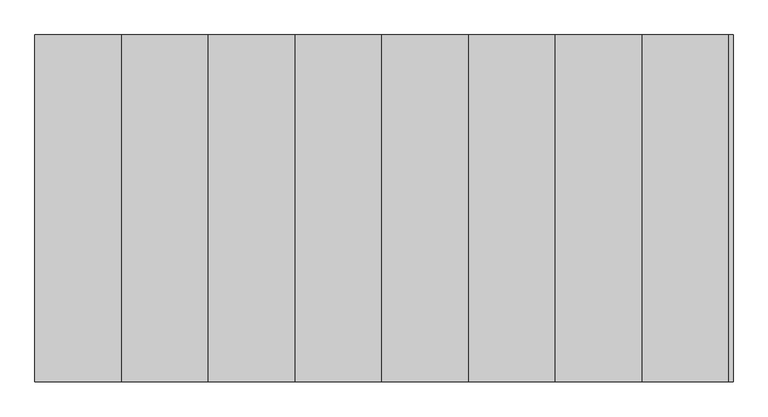
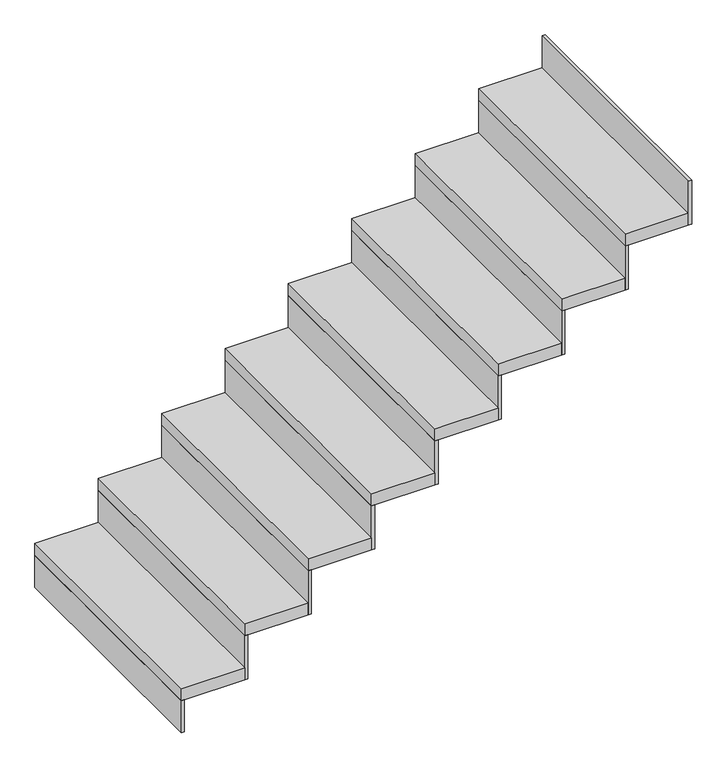
"""IFC4 building model written with IfcOpenShell, lengths in millimetres: stair flight geometry."""

from ifc_helpers import new_model, si_unit, frame, origin, origin_with_axes, place, context, project, spatial, polyline, outline, extrude, source, transform, mapped, element, save


def stair_flight_23111021(model_context):
    return source(origin(), model_context, "Body", "SweptSolid", [
        extrude(outline(polyline([(3289.0556606, 2685.7983707), (3276.5556606, 2685.7983707), (3276.5556606, 3685.7983707), (3289.0556606, 3685.7983707), (3289.0556606, 2685.7983707)])), origin_with_axes(), (0.0, 0.0, 1.0), 133.3333333),
        extrude(outline(polyline([(3526.5556606, 3685.7983707), (3526.5556606, 2685.7983707), (3276.5556606, 2685.7983707), (3276.5556606, 3685.7983707), (3526.5556606, 3685.7983707)])), frame((0.0, 0.0, 133.3333333), z_axis=(0.0, 0.0, 1.0), x_axis=(1.0, 0.0, 0.0)), (0.0, 0.0, 1.0), 50.0),
        extrude(outline(polyline([(3539.0556606, 2685.7983707), (3526.5556606, 2685.7983707), (3526.5556606, 3685.7983707), (3539.0556606, 3685.7983707), (3539.0556606, 2685.7983707)])), frame((0.0, 0.0, 133.3333333), z_axis=(0.0, 0.0, 1.0), x_axis=(1.0, 0.0, 0.0)), (0.0, 0.0, 1.0), 183.3333333),
        extrude(outline(polyline([(3776.5556606, 3685.7983707), (3776.5556606, 2685.7983707), (3526.5556606, 2685.7983707), (3526.5556606, 3685.7983707), (3776.5556606, 3685.7983707)])), frame((0.0, 0.0, 316.6666667), z_axis=(0.0, 0.0, 1.0), x_axis=(1.0, 0.0, 0.0)), (0.0, 0.0, 1.0), 50.0),
        extrude(outline(polyline([(3789.0556606, 2685.7983707), (3776.5556606, 2685.7983707), (3776.5556606, 3685.7983707), (3789.0556606, 3685.7983707), (3789.0556606, 2685.7983707)])), frame((0.0, 0.0, 316.6666667), z_axis=(0.0, 0.0, 1.0), x_axis=(1.0, 0.0, 0.0)), (0.0, 0.0, 1.0), 183.3333333),
        extrude(outline(polyline([(4026.5556606, 3685.7983707), (4026.5556606, 2685.7983707), (3776.5556606, 2685.7983707), (3776.5556606, 3685.7983707), (4026.5556606, 3685.7983707)])), frame((0.0, 0.0, 500.0), z_axis=(0.0, 0.0, 1.0), x_axis=(1.0, 0.0, 0.0)), (0.0, 0.0, 1.0), 50.0),
        extrude(outline(polyline([(4039.0556606, 2685.7983707), (4026.5556606, 2685.7983707), (4026.5556606, 3685.7983707), (4039.0556606, 3685.7983707), (4039.0556606, 2685.7983707)])), frame((0.0, 0.0, 500.0), z_axis=(0.0, 0.0, 1.0), x_axis=(1.0, 0.0, 0.0)), (0.0, 0.0, 1.0), 183.3333333),
        extrude(outline(polyline([(4276.5556606, 3685.7983707), (4276.5556606, 2685.7983707), (4026.5556606, 2685.7983707), (4026.5556606, 3685.7983707), (4276.5556606, 3685.7983707)])), frame((0.0, 0.0, 683.3333333), z_axis=(0.0, 0.0, 1.0), x_axis=(1.0, 0.0, 0.0)), (0.0, 0.0, 1.0), 50.0),
        extrude(outline(polyline([(4289.0556606, 2685.7983707), (4276.5556606, 2685.7983707), (4276.5556606, 3685.7983707), (4289.0556606, 3685.7983707), (4289.0556606, 2685.7983707)])), frame((0.0, 0.0, 683.3333333), z_axis=(0.0, 0.0, 1.0), x_axis=(1.0, 0.0, 0.0)), (0.0, 0.0, 1.0), 183.3333333),
        extrude(outline(polyline([(4526.5556606, 3685.7983707), (4526.5556606, 2685.7983707), (4276.5556606, 2685.7983707), (4276.5556606, 3685.7983707), (4526.5556606, 3685.7983707)])), frame((0.0, 0.0, 866.6666667), z_axis=(0.0, 0.0, 1.0), x_axis=(1.0, 0.0, 0.0)), (0.0, 0.0, 1.0), 50.0),
        extrude(outline(polyline([(4539.0556606, 2685.7983707), (4526.5556606, 2685.7983707), (4526.5556606, 3685.7983707), (4539.0556606, 3685.7983707), (4539.0556606, 2685.7983707)])), frame((0.0, 0.0, 866.6666667), z_axis=(0.0, 0.0, 1.0), x_axis=(1.0, 0.0, 0.0)), (0.0, 0.0, 1.0), 183.3333333),
        extrude(outline(polyline([(4776.5556606, 3685.7983707), (4776.5556606, 2685.7983707), (4526.5556606, 2685.7983707), (4526.5556606, 3685.7983707), (4776.5556606, 3685.7983707)])), frame((0.0, 0.0, 1050.0), z_axis=(0.0, 0.0, 1.0), x_axis=(1.0, 0.0, 0.0)), (0.0, 0.0, 1.0), 50.0),
        extrude(outline(polyline([(4789.0556606, 2685.7983707), (4776.5556606, 2685.7983707), (4776.5556606, 3685.7983707), (4789.0556606, 3685.7983707), (4789.0556606, 2685.7983707)])), frame((0.0, 0.0, 1050.0), z_axis=(0.0, 0.0, 1.0), x_axis=(1.0, 0.0, 0.0)), (0.0, 0.0, 1.0), 183.3333333),
        extrude(outline(polyline([(5026.5556606, 3685.7983707), (5026.5556606, 2685.7983707), (4776.5556606, 2685.7983707), (4776.5556606, 3685.7983707), (5026.5556606, 3685.7983707)])), frame((0.0, 0.0, 1233.3333333), z_axis=(0.0, 0.0, 1.0), x_axis=(1.0, 0.0, 0.0)), (0.0, 0.0, 1.0), 50.0),
        extrude(outline(polyline([(5039.0556606, 2685.7983707), (5026.5556606, 2685.7983707), (5026.5556606, 3685.7983707), (5039.0556606, 3685.7983707), (5039.0556606, 2685.7983707)])), frame((0.0, 0.0, 1233.3333333), z_axis=(0.0, 0.0, 1.0), x_axis=(1.0, 0.0, 0.0)), (0.0, 0.0, 1.0), 183.3333333),
        extrude(outline(polyline([(5289.0556606, 2685.7983707), (5276.5556606, 2685.7983707), (5276.5556606, 3685.7983707), (5289.0556606, 3685.7983707), (5289.0556606, 2685.7983707)])), frame((0.0, 0.0, 1416.6666667), z_axis=(0.0, 0.0, 1.0), x_axis=(1.0, 0.0, 0.0)), (0.0, 0.0, 1.0), 183.3333333),
        extrude(outline(polyline([(5276.5556606, 3685.7983707), (5276.5556606, 2685.7983707), (5026.5556606, 2685.7983707), (5026.5556606, 3685.7983707), (5276.5556606, 3685.7983707)])), frame((0.0, 0.0, 1416.6666667), z_axis=(0.0, 0.0, 1.0), x_axis=(1.0, 0.0, 0.0)), (0.0, 0.0, 1.0), 50.0),
    ])


if __name__ == "__main__":
    model = new_model("IFC4")
    model_context = context("Model", 3, world=origin())
    ifc_project = project(units=[si_unit("LENGTHUNIT", "METRE", prefix="MILLI")], contexts=[model_context])
    site = spatial("IfcSite", under=ifc_project)
    building = spatial("IfcBuilding", under=site)
    placement = place(None, origin())
    stair_flight_shape = stair_flight_23111021(model_context)
    element("IfcStairFlight", 1, at=placement, inside=building, context=model_context, shape_type="MappedRepresentation", body=[
        mapped(stair_flight_shape, transform((0.0, 0.0, 0.0), x_axis=(1.0, 0.0, 0.0), y_axis=(0.0, 1.0, 0.0), z_axis=(0.0, 0.0, 1.0))),
    ])
    save(model, "model.ifc")
